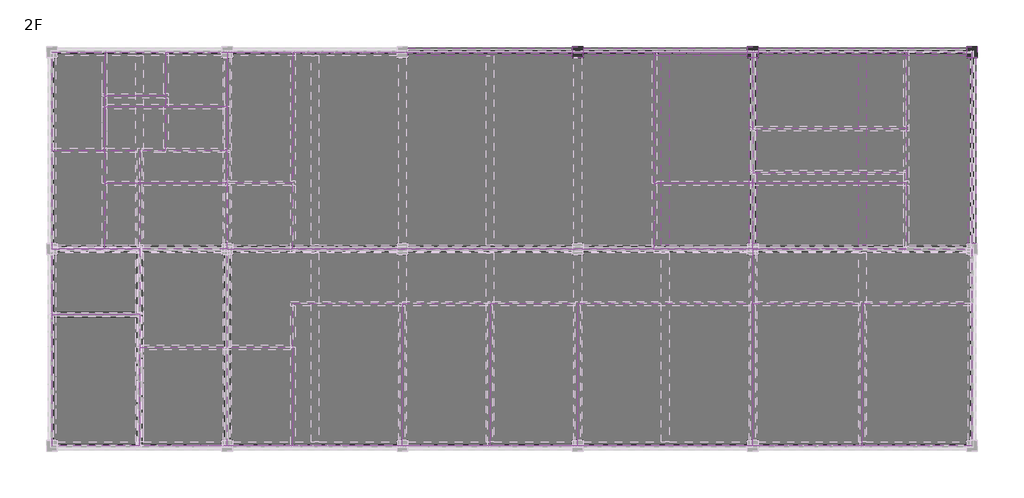
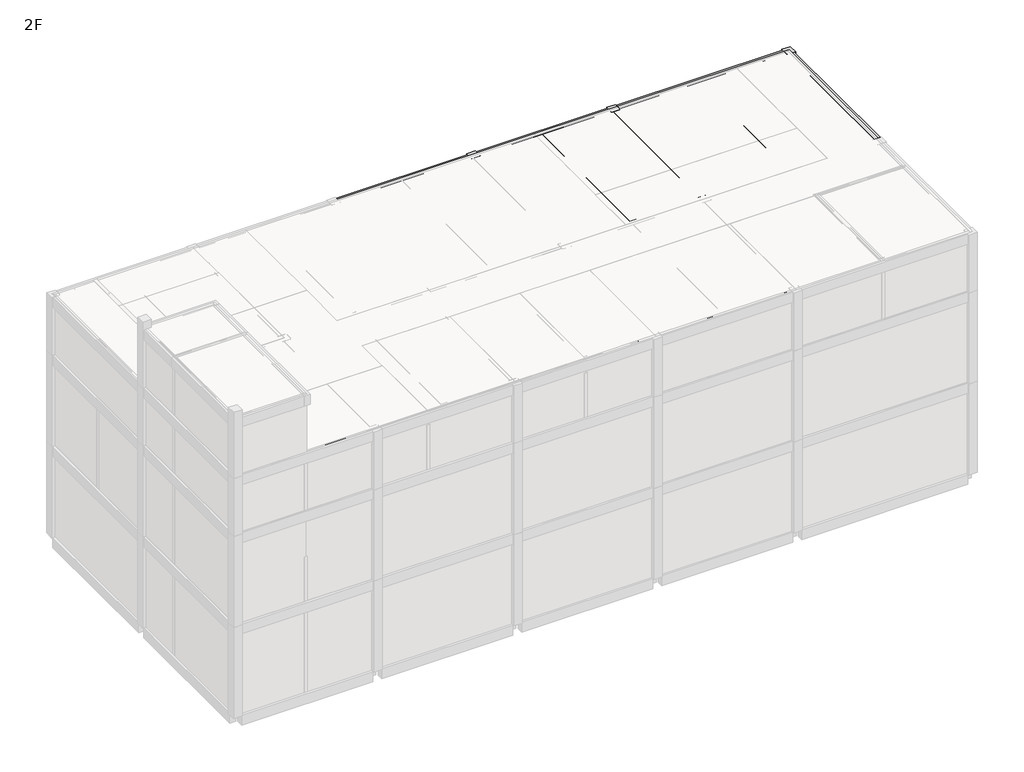
# One storey, part 7 of 7: 39 proxies, 28 beams, 9 columns.
# Revit data of these elements (continued)
# Type "Concrete-Rectangular-Beam : BM111_400x500_RG1"
#   중앙부 하부근 = "3-D20"
#   중앙부 상부근 = "3-D20"
#   중앙부 보조근 = ""
#   중앙부 늑근 = "2-D10 @200"
#   외단부 하부근 = "3-D20"
#   외단부 상부근 = "3-D20"
#   외단부 보조근 = ""
#   외단부 늑근 = "2-D10 @100"
#   부호 = "RG1"
#   내단부 하부근 = "3-D20"
#   내단부 상부근 = "3-D20"
#   내단부 보조근 = ""
#   내단부 늑근 = "2-D10 @100"
#   ALL 하부근 = ""
#   ALL 상부근 = ""
#   ALL 보조근 = ""
#   ALL 늑근 = ""
#   Width = 400 mm
#   Height = 500 mm
#   Length [instance default] = 1524 mm
#   Structural Material [instance default] = 콘크리트 - 현장타설 콘크리트
#   hec_material3 [instance default] = none
#   hec_material2 [instance default] = none
#   hec_material1 [instance default] = none
#   Assembly Code = ""
# Type "Space Planning Box_hec : Space Planning Box_hec"
#   Type Comments = "..."
#   Room Name [instance default] = "?"
#   Interior Finish [instance default] = ""
#   Exterior Finish [instance default] = ""
#   Department [instance default] = ""
#   Assembly Code = "..."
#   ceiling height [instance default] = 0
#   Width [instance default] = 1524 mm
#   Program Area [instance default] = 0.00 m²
#   Length [instance default] = 1524 mm
#   Height [instance default] = 1524 mm
#   Area [instance default] = 2.32258 m²
#   Fill Color [instance default] = Cyan
#   Default Elevation = 0
# Type "Concrete-Rectangular-Column : CL111_500x500"
#   Description = "UG 철골 기둥용 Pedestal"
#   b = 500 mm
#   h = 500 mm
#   hec_material3 [instance default] = none
#   hec_material2 [instance default] = A03AE056-00001_Bitumen/Bituminous/Asphalt Coating
#   hec_material1 [instance default] = A03AC035-00001_Form Work (3 times in use)_Flat
#   Structural Material [instance default] = A03AC032-00007_Structural Concrete_Type1_25MPa-30Mpa
# Elements 1, 2, 3, 4, 5, 6, 7, 8, 9, 10, 11, 12, 13, 14, 15, 16, 17, 18, 19, 20, 21, 22, 23, 24, 25, 26, 27, 28 (IfcBeam, "Concrete-Rectangular-Beam : BM111_400x500_RG1")
#   Comments = ""
#   hec_material3 = none
#   hec_material2 = none
#   hec_material1 = none
#   Structural Material = 콘크리트 - 현장타설 콘크리트
#   Phase Created = New Construction
#   Materials on its faces: "콘크리트 - 현장타설 콘크리트"
# Element 29 (IfcBuildingElementProxy, "Space Planning Box_hec : Space Planning Box_hec")
#   Room Name = "Staircase"
#   Interior Finish = "IW5..N/A..N/A,,N/A..N/A,,FL2..N/A,,CL1..N/A"
#   Exterior Finish = "N/A..N/A,,EW2..N/A..N/A"
#   Department = "PATHV1"
#   ceiling height = 0
#   Width = 4000 mm
#   Program Area = 24.00 m²
#   Length = 6000 mm
#   Height = 3500 mm
#   Area = 24.00 m²
#   Fill Color = Green
#   Phase Created = New Construction
#   Materials on its faces: "Green"
# Element 30 (IfcBuildingElementProxy, "Space Planning Box_hec : Space Planning Box_hec")
#   Room Name = "Staircase"
#   Interior Finish = "IW5..N/A..N/A,,WK3..N/A,,FL2..N/A,,CL1..N/A"
#   Exterior Finish = "RF1..N/A,,EW2..EW1..N/A"
#   Department = "PATHV1"
#   ceiling height = 0
#   Width = 4000 mm
#   Program Area = 0.00 m²
#   Length = 6000 mm
#   Height = 3500 mm
#   Area = 24.00 m²
#   Fill Color = Green
#   Phase Created = New Construction
#   Materials on its faces: "Green"
# Element 31 (IfcBuildingElementProxy, "Space Planning Box_hec : Space Planning Box_hec")
#   Room Name = "Electrical Room-1"
#   Interior Finish = "IW5..N/A..N/A,,WK1..N/A,,FL1..N/A,,CL1..N/A"
#   Exterior Finish = "N/A..N/A,,EW1..EW2..N/A"
#   Department = "CI"
#   ceiling height = 0
#   Width = 9000 mm
#   Program Area = 306.00 m²
#   Length = 32000 mm
#   Height = 5500 mm
#   Area = 288.00 m²
#   Fill Color = Yellow
#   Phase Created = New Construction
#   Materials on its faces: "Yellow"
# Element 32 (IfcBuildingElementProxy, "Space Planning Box_hec : Space Planning Box_hec")
#   Room Name = "Electrical Room-2"
#   Interior Finish = "IW5..N/A..N/A,,WK1..N/A,,FL1..N/A,,CL1..N/A"
#   Exterior Finish = "N/A..N/A,,EW1..EW2..N/A"
#   Department = "EL"
#   ceiling height = 0
#   Width = 9000 mm
#   Program Area = 288.00 m²
#   Length = 34000 mm
#   Height = 5500 mm
#   Area = 306.00 m²
#   Fill Color = Orange
#   Phase Created = New Construction
#   Materials on its faces: "Orange"
# Element 33 (IfcBuildingElementProxy, "Space Planning Box_hec : Space Planning Box_hec")
#   Room Name = "Electrical Room (GIS)"
#   Interior Finish = "IW5..N/A..N/A,,WK1..N/A,,FL1..N/A,,CL1..N/A"
#   Exterior Finish = "N/A..N/A,,EW1..EW2..N/A"
#   Department = "AR"
#   ceiling height = 0
#   Width = 9000 mm
#   Program Area = 90.00 m²
#   Length = 10000 mm
#   Height = 5500 mm
#   Area = 90.00 m²
#   Fill Color = Cyan
#   Phase Created = New Construction
#   Materials on its faces: "Cyan"
# Element 34 (IfcBuildingElementProxy, "Space Planning Box_hec : Space Planning Box_hec")
#   Room Name = "Lobby"
#   Interior Finish = "IW5..N/A..N/A,,WK3..N/A,,FL2..N/A,,CL3..N/A"
#   Exterior Finish = "N/A..N/A,,EW2..N/A..N/A"
#   Department = "AR"
#   ceiling height = 2700
#   Width = 4000 mm
#   Program Area = 36.00 m²
#   Length = 9000 mm
#   Height = 5500 mm
#   Area = 36.00 m²
#   Fill Color = Cyan
#   Phase Created = New Construction
#   Materials on its faces: "Cyan"
# Elements 35, 36 (IfcBuildingElementProxy, "Space Planning Box_hec : Space Planning Box_hec")
#   Room Name = "Elevator"
#   Interior Finish = "N/A..N/A..N/A,,N/A..N/A,,N/A..N/A,,N/A..N/A"
#   Exterior Finish = "N/A..N/A,,EW2..N/A..N/A"
#   Department = "PATHV2"
#   ceiling height = 0
#   Width = 4000 mm
#   Program Area = 12.00 m²
#   Length = 3000 mm
#   Height = 5500 mm
#   Area = 12.00 m²
#   Fill Color = Blue
#   Phase Created = New Construction
#   Materials on its faces: "Blue"
# Element 37 (IfcBuildingElementProxy, "Space Planning Box_hec : Space Planning Box_hec")
#   Room Name = "Staircase"
#   Interior Finish = "IW5..N/A..N/A,,WK3..N/A,,FL2..N/A,,CL1..N/A"
#   Exterior Finish = "N/A..N/A,,EW2..N/A..N/A"
#   Department = "PATHV1"
#   ceiling height = 0
#   Width = 4000 mm
#   Program Area = 24.00 m²
#   Length = 6000 mm
#   Height = 5500 mm
#   Area = 24.00 m²
#   Fill Color = Green
#   Phase Created = New Construction
#   Materials on its faces: "Green"
# Element 38 (IfcBuildingElementProxy, "Space Planning Box_hec : Space Planning Box_hec")
#   Room Name = "Staircase"
#   Interior Finish = "IW5..N/A..N/A,,WK3..N/A,,FL2..N/A,,CL1..N/A"
#   Exterior Finish = "N/A..N/A,,EW2..N/A..N/A"
#   Department = "PATHV1"
#   ceiling height = 2700
#   Width = 4000 mm
#   Program Area = 24.00 m²
#   Length = 6000 mm
#   Height = 5500 mm
#   Area = 24.00 m²
#   Fill Color = Green
#   Phase Created = New Construction
#   Materials on its faces: "Green"
# Element 39 (IfcBuildingElementProxy, "Space Planning Box_hec : Space Planning Box_hec")
#   Room Name = "Central Control Room"
#   Interior Finish = "IW5..N/A..N/A,,N/A..N/A,,FL5..N/A,,CL3..N/A"
#   Exterior Finish = "N/A..N/A,,EW1..N/A..N/A"
#   Department = "CI"
#   ceiling height = 3400
#   Width = 9000 mm
#   Program Area = 216.00 m²
#   Length = 24000 mm
#   Height = 5500 mm
#   Area = 216.00 m²
#   Fill Color = Yellow
#   Phase Created = New Construction
#   Materials on its faces: "Yellow"
# Element 40 (IfcBuildingElementProxy, "Space Planning Box_hec : Space Planning Box_hec")
#   Room Name = "Electronic Room"
#   Interior Finish = "IW5..N/A..N/A,,N/A..N/A,,FL5..N/A,,CL3..N/A"
#   Exterior Finish = "N/A..N/A,,EW1..N/A..N/A"
#   Department = "CI"
#   ceiling height = 3000
#   Width = 9000 mm
#   Program Area = 216.00 m²
#   Length = 24000 mm
#   Height = 5500 mm
#   Area = 216.00 m²
#   Fill Color = Yellow
#   Phase Created = New Construction
#   Materials on its faces: "Yellow"
# Element 41 (IfcBuildingElementProxy, "Space Planning Box_hec : Space Planning Box_hec")
#   Room Name = "Computer Room"
#   Interior Finish = "IW5..N/A..N/A,,N/A..N/A,,FL5..N/A,,CL3..N/A"
#   Exterior Finish = "N/A..N/A,,EW2..N/A..N/A"
#   Department = "AR"
#   ceiling height = 2700
#   Width = 7000 mm
#   Program Area = 24.50 m²
#   Length = 3500 mm
#   Height = 5500 mm
#   Area = 24.50 m²
#   Fill Color = Cyan
#   Phase Created = New Construction
#   Materials on its faces: "Cyan"
# Element 42 (IfcBuildingElementProxy, "Space Planning Box_hec : Space Planning Box_hec")
#   Room Name = "Electrical Room -3"
#   Interior Finish = "IW5..N/A..N/A,,N/A..N/A,,FL5,,CL3..N/A"
#   Exterior Finish = "N/A..N/A,,EW2..N/A..N/A"
#   Department = "EL"
#   ceiling height = 0
#   Width = 9000 mm
#   Program Area = 90.00 m²
#   Length = 10000 mm
#   Height = 5500 mm
#   Area = 90.00 m²
#   Fill Color = Orange
#   Phase Created = New Construction
#   Materials on its faces: "Orange"
# Element 43 (IfcBuildingElementProxy, "Space Planning Box_hec : Space Planning Box_hec")
#   Room Name = "Communication Room"
#   Interior Finish = "IW5..N/A..N/A,,N/A..N/A,,FL5..N/A,,CL3..N/A"
#   Exterior Finish = "N/A..N/A,,N/A..N/A..N/A"
#   Department = "CI"
#   ceiling height = 2700
#   Width = 7000 mm
#   Program Area = 24.50 m²
#   Length = 3500 mm
#   Height = 5500 mm
#   Area = 24.50 m²
#   Fill Color = Yellow
#   Phase Created = New Construction
#   Materials on its faces: "Yellow"
# Element 44 (IfcBuildingElementProxy, "Space Planning Box_hec : Space Planning Box_hec")
#   Room Name = "Duct Shaft"
#   Interior Finish = "N/A..N/A..N/A,,N/A..N/A,,N/A..N/A,,N/A..N/A"
#   Exterior Finish = "N/A..N/A,,EW2..N/A..N/A"
#   Department = "PATHV3"
#   ceiling height = 0
#   Width = 2400 mm
#   Program Area = 10.80 m²
#   Length = 4500 mm
#   Height = 5500 mm
#   Area = 10.80 m²
#   Fill Color = Lavender
#   Phase Created = New Construction
#   Materials on its faces: "Lavender"
# Element 45 (IfcBuildingElementProxy, "Space Planning Box_hec : Space Planning Box_hec")
#   Room Name = "Toilet (M)"
#   Interior Finish = "IW3..N/A..N/A,,N/A..N/A,,FL3..N/A,,CL4..N/A"
#   Exterior Finish = "N/A..N/A,,EW2..N/A..N/A"
#   Department = "AR"
#   ceiling height = 2700
#   Width = 4000 mm
#   Program Area = 18.00 m²
#   Length = 4500 mm
#   Height = 5500 mm
#   Area = 18.00 m²
#   Fill Color = Cyan
#   Phase Created = New Construction
#   Materials on its faces: "Cyan"
# Element 46 (IfcBuildingElementProxy, "Space Planning Box_hec : Space Planning Box_hec")
#   Room Name = "Toilet"
#   Interior Finish = "IW3..N/A..N/A,,N/A..N/A,,FL3..N/A,,CL4..N/A"
#   Exterior Finish = "N/A..N/A,,EW2..N/A..N/A"
#   Department = "AR"
#   ceiling height = 2700
#   Width = 2800 mm
#   Program Area = 12.60 m²
#   Length = 4500 mm
#   Height = 5500 mm
#   Area = 12.60 m²
#   Fill Color = Cyan
#   Phase Created = New Construction
#   Materials on its faces: "Cyan"
# Element 47 (IfcBuildingElementProxy, "Space Planning Box_hec : Space Planning Box_hec")
#   Room Name = "Shower"
#   Interior Finish = "IW3..N/A..N/A,,N/A..N/A,,FL3..N/A,,CL4..N/A"
#   Exterior Finish = "N/A..N/A,,EW2..N/A..N/A"
#   Department = "AR"
#   ceiling height = 2700
#   Width = 2800 mm
#   Program Area = 5.60 m²
#   Length = 2000 mm
#   Height = 5500 mm
#   Area = 5.60 m²
#   Fill Color = Cyan
#   Phase Created = New Construction
#   Materials on its faces: "Cyan"
# Element 48 (IfcBuildingElementProxy, "Space Planning Box_hec : Space Planning Box_hec")
#   Room Name = "Locker(F)"
#   Interior Finish = "IW5..N/A..N/A,,WK3..N/A,,FL2..N/A,,CL3..N/A"
#   Exterior Finish = "N/A..N/A,,N/A..N/A..N/A"
#   Department = "AR"
#   ceiling height = 2700
#   Width = 2800 mm
#   Program Area = 7.00 m²
#   Length = 2500 mm
#   Height = 5500 mm
#   Area = 7.00 m²
#   Fill Color = Cyan
#   Phase Created = New Construction
#   Materials on its faces: "Cyan"
# Element 49 (IfcBuildingElementProxy, "Space Planning Box_hec : Space Planning Box_hec")
#   Room Name = "Manager Office-1"
#   Interior Finish = "IW5..N/A..N/A,,WK3..N/A,,FL2..N/A,,CL3..N/A"
#   Exterior Finish = "RF1..N/A,,EW1..N/A..N/A"
#   Department = "AR"
#   ceiling height = 2700
#   Width = 6500 mm
#   Program Area = 26.00 m²
#   Length = 4000 mm
#   Height = 3500 mm
#   Area = 26.00 m²
#   Fill Color = Cyan
#   Phase Created = New Construction
#   Materials on its faces: "Cyan"
# Element 50 (IfcBuildingElementProxy, "Space Planning Box_hec : Space Planning Box_hec")
#   Room Name = "Manager Office-2"
#   Interior Finish = "IW5..N/A..N/A,,WK3..N/A,,FL2..N/A,,CL3..N/A"
#   Exterior Finish = "RF1..N/A,,EW1..N/A..N/A"
#   Department = "AR"
#   ceiling height = 2700
#   Width = 6500 mm
#   Program Area = 26.00 m²
#   Length = 4000 mm
#   Height = 3500 mm
#   Area = 26.00 m²
#   Fill Color = Cyan
#   Phase Created = New Construction
#   Materials on its faces: "Cyan"
# Element 51 (IfcBuildingElementProxy, "Space Planning Box_hec : Space Planning Box_hec")
#   Room Name = "Meeting Room-1"
#   Interior Finish = "IW5..N/A..N/A,,WK3..N/A,,FL2..N/A,,CL3..N/A"
#   Exterior Finish = "RF1..N/A,,EW1..EW2..N/A"
#   Department = "AR"
#   ceiling height = 2700
#   Width = 6000 mm
#   Program Area = 69.00 m²
#   Length = 11500 mm
#   Height = 3500 mm
#   Area = 69.00 m²
#   Fill Color = Cyan
#   Phase Created = New Construction
#   Materials on its faces: "Cyan"
# Element 52 (IfcBuildingElementProxy, "Space Planning Box_hec : Space Planning Box_hec")
#   Room Name = "Meeting Room-2"
#   Interior Finish = "IW5..N/A..N/A,,WK3..N/A,,FL2..N/A,,CL3..N/A"
#   Exterior Finish = "RF1..N/A,,EW1..N/A..N/A"
#   Department = "AR"
#   ceiling height = 2700
#   Width = 6500 mm
#   Program Area = 52.00 m²
#   Length = 8000 mm
#   Height = 3500 mm
#   Area = 52.00 m²
#   Fill Color = Cyan
#   Phase Created = New Construction
#   Materials on its faces: "Cyan"
# Element 53 (IfcBuildingElementProxy, "Space Planning Box_hec : Space Planning Box_hec")
#   Room Name = "Open Office"
#   Interior Finish = "IW5..N/A..N/A,,WK3..N/A,,FL2..N/A,,CL3..N/A"
#   Exterior Finish = "RF1..N/A,,EW1..N/A..N/A"
#   Department = "HV"
#   ceiling height = 2700
#   Width = 9000 mm
#   Program Area = 148.50 m²
#   Length = 16500 mm
#   Height = 3500 mm
#   Area = 148.50 m²
#   Fill Color = Lime
#   Phase Created = New Construction
#   Materials on its faces: "Lime"
# Element 54 (IfcBuildingElementProxy, "Space Planning Box_hec : Space Planning Box_hec")
#   Room Name = "Office-1"
#   Interior Finish = "IW5..N/A..N/A,,WK3..N/A,,FL2..N/A,,CL3..N/A"
#   Exterior Finish = "RF1..N/A,,EW2..N/A..N/A"
#   Department = "AR"
#   ceiling height = 2700
#   Width = 6500 mm
#   Program Area = 32.50 m²
#   Length = 5000 mm
#   Height = 3500 mm
#   Area = 32.50 m²
#   Fill Color = Cyan
#   Phase Created = New Construction
#   Materials on its faces: "Cyan"
# Element 55 (IfcBuildingElementProxy, "Space Planning Box_hec : Space Planning Box_hec")
#   Room Name = "Storage"
#   Interior Finish = "IW5..N/A..N/A,,WK3..N/A,,FL2..N/A,,CL3..N/A"
#   Exterior Finish = "RF1..N/A,,EW1..N/A..N/A"
#   Department = "AR"
#   ceiling height = 2700
#   Width = 6500 mm
#   Program Area = 32.50 m²
#   Length = 5000 mm
#   Height = 3500 mm
#   Area = 32.50 m²
#   Fill Color = Cyan
#   Phase Created = New Construction
#   Materials on its faces: "Cyan"
# Element 56 (IfcBuildingElementProxy, "Space Planning Box_hec : Space Planning Box_hec")
#   Room Name = "Fire Gas Room"
#   Interior Finish = "IW5..N/A..N/A,,WK1..N/A,,FL1..N/A,,N/A..N/A"
#   Exterior Finish = "RF1..N/A,,EW2..N/A..N/A"
#   Department = "FF"
#   ceiling height = 0
#   Width = 6500 mm
#   Program Area = 32.50 m²
#   Length = 5000 mm
#   Height = 3500 mm
#   Area = 32.50 m²
#   Fill Color = Red
#   Phase Created = New Construction
#   Materials on its faces: "Red"
# Element 57 (IfcBuildingElementProxy, "Space Planning Box_hec : Space Planning Box_hec")
#   Room Name = "Document Room"
#   Interior Finish = "IW5..N/A..N/A,,WK3..N/A,,FL2..N/A,,CL3..N/A"
#   Exterior Finish = "RF1..N/A,,N/A..N/A..N/A"
#   Department = "AR"
#   ceiling height = 2700
#   Width = 3000 mm
#   Program Area = 34.50 m²
#   Length = 11500 mm
#   Height = 3500 mm
#   Area = 34.50 m²
#   Fill Color = Cyan
#   Phase Created = New Construction
#   Materials on its faces: "Cyan"
# Element 58 (IfcBuildingElementProxy, "Space Planning Box_hec : Space Planning Box_hec")
#   Room Name = "Break Room"
#   Interior Finish = "IW5..N/A..N/A,,WK3..N/A,,FL2..N/A,,CL3..N/A"
#   Exterior Finish = "RF1..N/A,,EW2..N/A..N/A"
#   Department = "AR"
#   ceiling height = 2700
#   Width = 4500 mm
#   Program Area = 31.50 m²
#   Length = 7000 mm
#   Height = 3500 mm
#   Area = 31.50 m²
#   Fill Color = Cyan
#   Phase Created = New Construction
#   Materials on its faces: "Cyan"
# Element 59 (IfcBuildingElementProxy, "Space Planning Box_hec : Space Planning Box_hec")
#   Room Name = "Toilet"
#   Interior Finish = "IW3..N/A..N/A,,N/A..N/A,,FL3..N/A,,CL4..N/A"
#   Exterior Finish = "RF1..N/A,,N/A..N/A..N/A"
#   Department = "AR"
#   ceiling height = 2700
#   Width = 3500 mm
#   Program Area = 19.60 m²
#   Length = 5600 mm
#   Height = 3500 mm
#   Area = 19.60 m²
#   Fill Color = Cyan
#   Phase Created = New Construction
#   Materials on its faces: "Cyan"
# Element 60 (IfcBuildingElementProxy, "Space Planning Box_hec : Space Planning Box_hec")
#   Room Name = "Shower"
#   Interior Finish = "IW3..N/A..N/A,,N/A..N/A,,FL3..N/A,,CL4..N/A"
#   Exterior Finish = "RF1..N/A,,EW2..N/A..N/A"
#   Department = "AR"
#   ceiling height = 2700
#   Width = 2500 mm
#   Program Area = 14.00 m²
#   Length = 5600 mm
#   Height = 3500 mm
#   Area = 14.00 m²
#   Fill Color = Cyan
#   Phase Created = New Construction
#   Materials on its faces: "Cyan"
# Element 61 (IfcBuildingElementProxy, "Space Planning Box_hec : Space Planning Box_hec")
#   Room Name = "Locker(M)"
#   Interior Finish = "IW5..N/A..N/A,,WK3..N/A,,FL2..N/A,,CL3..N/A"
#   Exterior Finish = "RF1..N/A,,EW1..N/A..N/A"
#   Department = "AR"
#   ceiling height = 2700
#   Width = 6000 mm
#   Program Area = 18.00 m²
#   Length = 3000 mm
#   Height = 3500 mm
#   Area = 18.00 m²
#   Fill Color = Cyan
#   Phase Created = New Construction
#   Materials on its faces: "Cyan"
# Element 62 (IfcBuildingElementProxy, "Space Planning Box_hec : Space Planning Box_hec")
#   Room Name = "Toilet(F)"
#   Interior Finish = "IW3..N/A..N/A,,N/A..N/A,,FL3..N/A,,CL4..N/A"
#   Exterior Finish = "RF1..N/A,,N/A..N/A..N/A"
#   Department = "AR"
#   ceiling height = 2700
#   Width = 3000 mm
#   Program Area = 16.80 m²
#   Length = 5600 mm
#   Height = 3500 mm
#   Area = 16.80 m²
#   Fill Color = Cyan
#   Phase Created = New Construction
#   Materials on its faces: "Cyan"
# Element 63 (IfcBuildingElementProxy, "Space Planning Box_hec : Space Planning Box_hec")
#   Room Name = "Duct Shaft"
#   Interior Finish = "N/A..N/A..N/A,,N/A..N/A,,N/A..N/A,,N/A..N/A"
#   Exterior Finish = "RF1..N/A,,EW2..N/A..N/A"
#   Department = "PATHV3"
#   ceiling height = 0
#   Width = 2400 mm
#   Program Area = 21.60 m²
#   Length = 9000 mm
#   Height = 3500 mm
#   Area = 21.60 m²
#   Fill Color = Lavender
#   Phase Created = New Construction
#   Materials on its faces: "Lavender"
# Element 64 (IfcBuildingElementProxy, "Space Planning Box_hec : Space Planning Box_hec")
#   Room Name = "Elevator"
#   Interior Finish = "N/A..N/A..N/A,,N/A..N/A,,N/A..N/A,,N/A..N/A"
#   Exterior Finish = "N/A..N/A,,EW2..N/A..N/A"
#   Department = "PATHV2"
#   ceiling height = 0
#   Width = 4000 mm
#   Program Area = 12.00 m²
#   Length = 3000 mm
#   Height = 3500 mm
#   Area = 12.00 m²
#   Fill Color = Blue
#   Phase Created = New Construction
#   Materials on its faces: "Blue"
# Element 65 (IfcBuildingElementProxy, "Space Planning Box_hec : Space Planning Box_hec")
#   Room Name = "Elevator"
#   Interior Finish = "N/A..N/A..N/A,,N/A..N/A,,N/A..N/A,,N/A..N/A"
#   Exterior Finish = "RF1..N/A,,EW2..EW1..N/A"
#   Department = "PATHV2"
#   ceiling height = 0
#   Width = 4000 mm
#   Program Area = 0.00 m²
#   Length = 3000 mm
#   Height = 3500 mm
#   Area = 12.00 m²
#   Fill Color = Blue
#   Phase Created = New Construction
#   Materials on its faces: "Blue"
# Element 66 (IfcBuildingElementProxy, "Space Planning Box_hec : Space Planning Box_hec")
#   Room Name = "Corridor"
#   Interior Finish = "IW5..N/A..N/A,,WK3..N/A,,FL2..N/A,,CL3..N/A"
#   Exterior Finish = "N/A..N/A,,EW2..N/A..N/A"
#   Department = "AR"
#   ceiling height = 2700
#   Width = 42000 mm
#   Program Area = 54.00 m²
#   Length = 18000 mm
#   Height = 5500 mm
#   Area = 756.00 m²
#   Fill Color = Cyan
#   Phase Created = New Construction
#   Materials on its faces: "Cyan"
# Element 67 (IfcBuildingElementProxy, "Space Planning Box_hec : Space Planning Box_hec")
#   Room Name = "Corridor"
#   Interior Finish = "IW5..N/A..N/A,,WK3..N/A,,FL2..N/A,,CL3..N/A"
#   Exterior Finish = "RF1..N/A,,EW2..N/A..N/A"
#   Department = "AR"
#   ceiling height = 2700
#   Width = 18000 mm
#   Program Area = 95.00 m²
#   Length = 42000 mm
#   Height = 3500 mm
#   Area = 756.00 m²
#   Fill Color = Cyan
#   Phase Created = New Construction
#   Materials on its faces: "Cyan"
# Elements 68, 69, 70, 71, 72, 73, 74, 75, 76 (IfcColumn, "Concrete-Rectangular-Column : CL111_500x500")
#   Comments = ""
#   hec_material3 = none
#   hec_material2 = none
#   hec_material1 = none
#   Structural Material = 콘크리트 - 현장타설 콘크리트
#   Phase Created = New Construction
#   Materials on its faces: "콘크리트 - 현장타설 콘크리트"
# Materials
#   "콘크리트 - 현장타설 콘크리트": class "콘크리트", colour RGB 192 192 192, transparency 0
#   "Cyan": class "Generic", colour RGB 0 255 255, transparency 0.2, Cost = 0
#   "A03AE056-00001_Bitumen/Bituminous/Asphalt Coating": class "Generic", colour RGB 17 17 17, transparency 0, Description = "Damp-proofing", W00) Work Master Code = "A03AE056-00001", W01) Work Master_Lv1 = "Concrete Work", W02) Work Master_Lv2 = "Concrete Protective Coating (U/G)", W03) Work Master_Spec.1 = "Bitumen/Bituminous/Asphalt Coating", Cost = 0
#   "A03AC035-00001_Form Work (3 times in use)_Flat": class "Wood", colour RGB 149 120 74, transparency 0, Description = "Plywood", W00) Work Master Code = "A03AC035-00001", W01) Work Master_Lv1 = "Concrete Work", W02) Work Master_Lv2 = "Substructure Work", W03) Work Master_Spec.1 = "Form Work (3 times in use)", W04) Work Master_Spec.2 = "Flat Form", W05) Work Master_Spec.3 = "Dressed Lumber, Plywood or Steel Form(Wood Planks are not Allowed) incl. Chamfer", Cost = 0
#   "A03AC032-00007_Structural Concrete_Type1_25MPa-30Mpa": class "Concrete", colour RGB 176 176 176, transparency 0, Keynote = "09910.A1", Description = "Reinf. Conc.", W00) Work Master Code = "A03AC032-00007", W01) Work Master_Lv1 = "Concrete Work", W02) Work Master_Lv2 = "Substructure Work", W03) Work Master_Spec.1 = "Structural Concrete", W04) Work Master_Spec.2 = "Cement Type-1", W05) Work Master_Spec.3 = "25MPa < F'c (Cylinder Strength) ≤ 30MPa", Cost = 0
#   "Green": class "Generic", colour RGB 0 128 0, transparency 0.2, Cost = 0
#   "Yellow": class "Generic", colour RGB 255 255 0, transparency 0.2, Cost = 0
#   "Orange": class "Generic", colour RGB 255 165 0, transparency 0.2, Cost = 0
#   "Blue": class "Generic", colour RGB 0 0 255, transparency 0.2, Cost = 0
#   "Lavender": class "Generic", colour RGB 186 85 211, transparency 0.2, Cost = 0
#   "Lime": class "Generic", colour RGB 0 255 0, transparency 0.2, Cost = 0
#   "Red": class "Generic", colour RGB 255 0 0, transparency 0.2, Cost = 0
